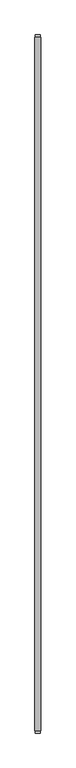
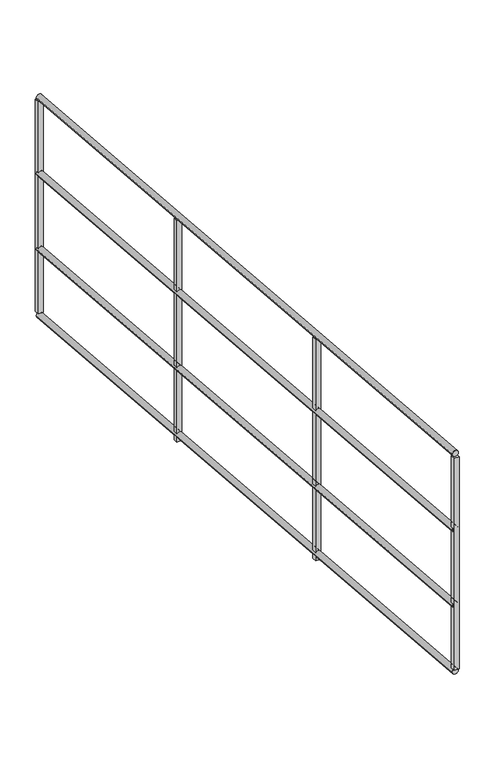
"""IFC4 building model written with IfcOpenShell, lengths in millimetres: railing geometry."""

from ifc_helpers import new_model, si_unit, frame, origin, place, context, project, spatial, polyline, ellipse_curve, outline, extrude, source, transform, mapped, element, save
from ifc_brep_helpers import plane_surface, cylinder_surface, advanced_brep


def railing_59a02c9f(model_context):
    return source(origin(), model_context, "Body", "SolidModel", [
        advanced_brep(
        [(20660.0, 22999.5208589, 1034.9098701), (20690.0, 22999.5208589, 1034.9098701), (20660.0, 19399.5208589, 1334.9098701), (20690.0, 19399.5208589, 1334.9098701)],
        [
            (0, 1, ellipse_curve(frame((20675.0, 22999.5208589, 1034.9098701), z_axis=(0.0, 1.0, 0.0), x_axis=(0.0, 0.0, -1.0)), 15.0519932, 15.0)),
            (1, 0, ellipse_curve(frame((20675.0, 22999.5208589, 1034.9098701), z_axis=(0.0, 1.0, 0.0), x_axis=(0.0, 0.0, -1.0)), 15.0519932, 15.0)),
            (2, 3, ellipse_curve(frame((20675.0, 19399.5208589, 1334.9098701), z_axis=(0.0, -1.0, 0.0), x_axis=(0.0, 0.0, -1.0)), 15.0519932, 15.0)),
            (3, 2, ellipse_curve(frame((20675.0, 19399.5208589, 1334.9098701), z_axis=(0.0, -1.0, 0.0), x_axis=(0.0, 0.0, -1.0)), 15.0519932, 15.0)),
            (0, 2),
            (3, 1),
        ],
        [
            plane_surface(frame((20675.0, 22999.5208589, 1049.9618634), z_axis=(0.0, 1.0, 0.0), x_axis=(0.0, 0.0, -1.0))),
            plane_surface(frame((20675.0, 19399.5208589, 1349.9618634), z_axis=(0.0, -1.0, 0.0), x_axis=(0.0, 0.0, -1.0))),
            cylinder_surface(frame((20675.0, 22998.2751767, 1035.013677), z_axis=(0.0, 0.9965457582448797, -0.08304547985373989), x_axis=(1.0, 0.0, 0.0)), 15.0),
        ],
        [
            (0, [[1, 2]]),
            (1, [[3, 4]]),
            (2, [[-1, 5, -4, 6]]),
            (2, [[-2, -6, -3, -5]]),
        ],
    ),
        advanced_brep(
        [(20660.0, 22999.5208589, 634.9098701), (20690.0, 22999.5208589, 634.9098701), (20660.0, 19399.5208589, 934.9098701), (20690.0, 19399.5208589, 934.9098701)],
        [
            (0, 1, ellipse_curve(frame((20675.0, 22999.5208589, 634.9098701), z_axis=(0.0, 1.0, 0.0), x_axis=(0.0, 0.0, -1.0)), 15.0519932, 15.0)),
            (1, 0, ellipse_curve(frame((20675.0, 22999.5208589, 634.9098701), z_axis=(0.0, 1.0, 0.0), x_axis=(0.0, 0.0, -1.0)), 15.0519932, 15.0)),
            (2, 3, ellipse_curve(frame((20675.0, 19399.5208589, 934.9098701), z_axis=(0.0, -1.0, 0.0), x_axis=(0.0, 0.0, -1.0)), 15.0519932, 15.0)),
            (3, 2, ellipse_curve(frame((20675.0, 19399.5208589, 934.9098701), z_axis=(0.0, -1.0, 0.0), x_axis=(0.0, 0.0, -1.0)), 15.0519932, 15.0)),
            (0, 2),
            (3, 1),
        ],
        [
            plane_surface(frame((20675.0, 22999.5208589, 649.9618634), z_axis=(0.0, 1.0, 0.0), x_axis=(0.0, 0.0, -1.0))),
            plane_surface(frame((20675.0, 19399.5208589, 949.9618634), z_axis=(0.0, -1.0, 0.0), x_axis=(0.0, 0.0, -1.0))),
            cylinder_surface(frame((20675.0, 22998.2751767, 635.013677), z_axis=(0.0, 0.9965457582448797, -0.08304547985373992), x_axis=(1.0, 0.0, 0.0)), 15.0),
        ],
        [
            (0, [[1, 2]]),
            (1, [[3, 4]]),
            (2, [[-1, 5, -4, 6]]),
            (2, [[-2, -6, -3, -5]]),
        ],
    ),
        advanced_brep(
        [(20660.0, 22999.5208589, 234.9098701), (20690.0, 22999.5208589, 234.9098701), (20660.0, 19399.5208589, 534.9098701), (20690.0, 19399.5208589, 534.9098701)],
        [
            (0, 1, ellipse_curve(frame((20675.0, 22999.5208589, 234.9098701), z_axis=(0.0, 1.0, 0.0), x_axis=(0.0, 0.0, -1.0)), 15.0519932, 15.0)),
            (1, 0, ellipse_curve(frame((20675.0, 22999.5208589, 234.9098701), z_axis=(0.0, 1.0, 0.0), x_axis=(0.0, 0.0, -1.0)), 15.0519932, 15.0)),
            (2, 3, ellipse_curve(frame((20675.0, 19399.5208589, 534.9098701), z_axis=(0.0, -1.0, 0.0), x_axis=(0.0, 0.0, -1.0)), 15.0519932, 15.0)),
            (3, 2, ellipse_curve(frame((20675.0, 19399.5208589, 534.9098701), z_axis=(0.0, -1.0, 0.0), x_axis=(0.0, 0.0, -1.0)), 15.0519932, 15.0)),
            (0, 2),
            (3, 1),
        ],
        [
            plane_surface(frame((20675.0, 22999.5208589, 249.9618634), z_axis=(0.0, 1.0, 0.0), x_axis=(0.0, 0.0, -1.0))),
            plane_surface(frame((20675.0, 19399.5208589, 549.9618634), z_axis=(0.0, -1.0, 0.0), x_axis=(0.0, 0.0, -1.0))),
            cylinder_surface(frame((20675.0, 22998.2751767, 235.013677), z_axis=(0.0, 0.9965457582448797, -0.08304547985373992), x_axis=(1.0, 0.0, 0.0)), 15.0),
        ],
        [
            (0, [[1, 2]]),
            (1, [[3, 4]]),
            (2, [[-1, 5, -4, 6]]),
            (2, [[-2, -6, -3, -5]]),
        ],
    ),
        advanced_brep(
        [(20660.0, 22999.5208589, -115.0901299), (20690.0, 22999.5208589, -115.0901299), (20660.0, 19399.5208589, 184.9098701), (20690.0, 19399.5208589, 184.9098701)],
        [
            (0, 1, ellipse_curve(frame((20675.0, 22999.5208589, -115.0901299), z_axis=(0.0, 1.0, 0.0), x_axis=(0.0, 0.0, -1.0)), 15.0519932, 15.0)),
            (1, 0, ellipse_curve(frame((20675.0, 22999.5208589, -115.0901299), z_axis=(0.0, 1.0, 0.0), x_axis=(0.0, 0.0, -1.0)), 15.0519932, 15.0)),
            (2, 3, ellipse_curve(frame((20675.0, 19399.5208589, 184.9098701), z_axis=(0.0, -1.0, 0.0), x_axis=(0.0, 0.0, -1.0)), 15.0519932, 15.0)),
            (3, 2, ellipse_curve(frame((20675.0, 19399.5208589, 184.9098701), z_axis=(0.0, -1.0, 0.0), x_axis=(0.0, 0.0, -1.0)), 15.0519932, 15.0)),
            (0, 2),
            (3, 1),
        ],
        [
            plane_surface(frame((20675.0, 22999.5208589, -100.0381366), z_axis=(0.0, 1.0, 0.0), x_axis=(0.0, 0.0, -1.0))),
            plane_surface(frame((20675.0, 19399.5208589, 199.9618634), z_axis=(0.0, -1.0, 0.0), x_axis=(0.0, 0.0, -1.0))),
            cylinder_surface(frame((20675.0, 22998.2751767, -114.986323), z_axis=(0.0, 0.9965457582448797, -0.08304547985373992), x_axis=(1.0, 0.0, 0.0)), 15.0),
        ],
        [
            (0, [[1, 2]]),
            (1, [[3, 4]]),
            (2, [[-1, 5, -4, 6]]),
            (2, [[-2, -6, -3, -5]]),
        ],
    ),
        extrude(outline(polyline([(20612.0208589, 48.9201967), (20587.0208589, 51.00353), (20587.0208589, 1220.8995436), (20612.0208589, 1218.8162103), (20612.0208589, 48.9201967)])), frame((20662.5, 0.0, 0.0), z_axis=(1.0, 0.0, 0.0), x_axis=(0.0, 1.0, 0.0)), (0.0, 0.0, 1.0), 25.0),
        extrude(outline(polyline([(21812.0208589, -51.0798033), (21787.0208589, -48.99647), (21787.0208589, 1120.8995436), (21812.0208589, 1118.8162103), (21812.0208589, -51.0798033)])), frame((20662.5, 0.0, 0.0), z_axis=(1.0, 0.0, 0.0), x_axis=(0.0, 1.0, 0.0)), (0.0, 0.0, 1.0), 25.0),
        extrude(outline(polyline([(19412.0208589, 198.9201967), (19387.0208589, 201.00353), (19387.0208589, 1320.8995436), (19412.0208589, 1318.8162103), (19412.0208589, 198.9201967)])), frame((20662.5, 0.0, 0.0), z_axis=(1.0, 0.0, 0.0), x_axis=(0.0, 1.0, 0.0)), (0.0, 0.0, 1.0), 25.0),
        extrude(outline(polyline([(23012.0208589, -101.0798033), (22987.0208589, -98.99647), (22987.0208589, 1020.8995436), (23012.0208589, 1018.8162103), (23012.0208589, -101.0798033)])), frame((20662.5, 0.0, 0.0), z_axis=(1.0, 0.0, 0.0), x_axis=(0.0, 1.0, 0.0)), (0.0, 0.0, 1.0), 25.0),
    ])


if __name__ == "__main__":
    model = new_model("IFC4")
    model_context = context("Model", 3, world=origin())
    ifc_project = project(units=[si_unit("LENGTHUNIT", "METRE", prefix="MILLI")], contexts=[model_context])
    site = spatial("IfcSite", under=ifc_project)
    building = spatial("IfcBuilding", under=site)
    placement = place(None, origin())
    railing_shape = railing_59a02c9f(model_context)
    element("IfcRailing", 1, at=placement, inside=building, context=model_context, shape_type="MappedRepresentation", body=[
        mapped(railing_shape, transform((0.0, 0.0, 0.0), x_axis=(1.0, 0.0, 0.0), y_axis=(0.0, 1.0, 0.0), z_axis=(0.0, 0.0, 1.0))),
    ])
    save(model, "model.ifc")
